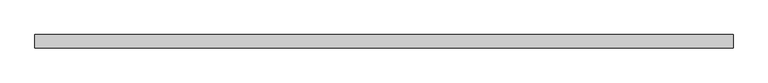
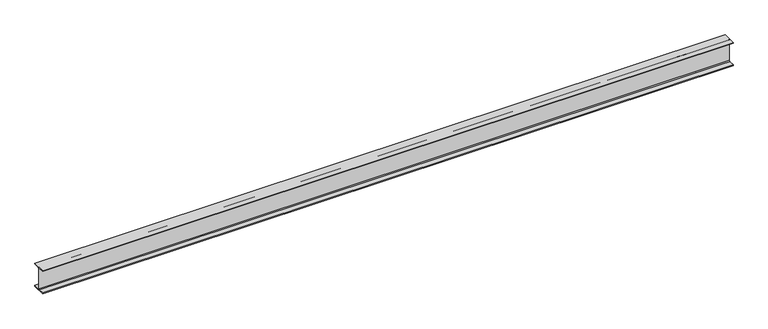
"""IFC4 building model written with IfcOpenShell, lengths in millimetres: beam geometry, Old_Steel Beam_H-KSD3502 : H_SB_ASB_H-300×300x10x15."""

from ifc_helpers import new_model, si_unit, point, frame, frame_2d, origin, place, context, project, spatial, polyline, circle_curve, trimmed, segment, composite_curve, outline, extrude, source, transform, mapped, element, save


def beam_082897f1(model_context):
    return source(origin(), model_context, "Body", "SweptSolid", [
        extrude(outline(composite_curve([segment(polyline([(82.5, -141.5), (82.5, -151.7), (-82.5, -151.7), (-82.5, -141.5), (-11.9, -141.5)]), True, "CONTINUOUS"), segment(trimmed(circle_curve(frame_2d((-11.9, -132.6)), 8.9), [point((-11.9, -141.5))], [point((-3.0, -132.6))], True, "CARTESIAN"), True, "CONTINUOUS"), segment(polyline([(-3.0, -132.6), (-3.0, 132.6)]), True, "CONTINUOUS"), segment(trimmed(circle_curve(frame_2d((-11.9, 132.6)), 8.9), [point((-3.0, 132.6))], [point((-11.9, 141.5))], True, "CARTESIAN"), True, "CONTINUOUS"), segment(polyline([(-11.9, 141.5), (-82.5, 141.5), (-82.5, 151.7), (82.5, 151.7), (82.5, 141.5), (11.9, 141.5)]), True, "CONTINUOUS"), segment(trimmed(circle_curve(frame_2d((11.9, 132.6)), 8.9), [point((11.9, 141.5))], [point((3.0, 132.6))], True, "CARTESIAN"), True, "CONTINUOUS"), segment(polyline([(3.0, 132.6), (3.0, -132.6)]), True, "CONTINUOUS"), segment(trimmed(circle_curve(frame_2d((11.9, -132.6)), 8.9), [point((3.0, -132.6))], [point((11.9, -141.5))], True, "CARTESIAN"), True, "CONTINUOUS"), segment(polyline([(11.9, -141.5), (82.5, -141.5)]), True, "CONTINUOUS")], self_intersect=False)), frame((-4272.9251782, 0.0, 0.0), z_axis=(1.0, 0.0, 0.0), x_axis=(0.0, 1.0, 0.0)), (0.0, 0.0, 1.0), 8596.9210734),
    ])


if __name__ == "__main__":
    model = new_model("IFC4")
    model_context = context("Model", 3, world=origin())
    ifc_project = project(units=[si_unit("LENGTHUNIT", "METRE", prefix="MILLI")], contexts=[model_context])
    site = spatial("IfcSite", under=ifc_project)
    building = spatial("IfcBuilding", under=site)
    placement = place(None, origin())
    beam_shape = beam_082897f1(model_context)
    element("IfcBeam", 1, ObjectType="Old_Steel Beam_H-KSD3502 : H_SB_ASB_H-300×300x10x15", at=placement, inside=building, context=model_context, shape_type="MappedRepresentation", body=[
        mapped(beam_shape, transform((0.0, 0.0, 0.0), x_axis=(1.0, 0.0, 0.0), y_axis=(0.0, 1.0, 0.0), z_axis=(0.0, 0.0, 1.0))),
    ])
    save(model, "model.ifc")

# Revit data of these elements
# Type "Old_Steel Beam_H-KSD3502 : H_SB_ASB_H-300×300x10x15"
#   Width = 30.0 cm
#   Web Thickness = 1.0 cm
#   Web Fillet = 1.8 cm
#   Warping Constant = 1370670.0 cm⁶
#   Torsional Moment of Inertia = 77.00 cm⁴
#   Torsional Modulus = 1.0 cm³
#   Section Area = 119.8 cm²
#   Plastic Modulus weak axis = 684.0 cm³
#   Plastic Modulus strong axis = 1500.0 cm³
#   Perimeter = 1.75 m²/m
#   Nominal Weight = 94.00 kgf/m
#   Moment of Inertia weak axis = 6750.00 cm⁴
#   Moment of Inertia strong axis = 20400.00 cm⁴
#   Height = 30.0 cm
#   Flange Thickness = 1.5 cm
#   Elastic Modulus weak axis = 450.0 cm³
#   Elastic Modulus strong axis = 1360.0 cm³
#   Centroid Vertical = 15.0 cm
#   Centroid Horizontal = 15.0 cm
#   Length [instance default] = 1.5240 m
#   Structural Material [instance default] = Steel, 45-345
#   Assembly Code = ""
# Element 1 (IfcBeam, "Old_Steel Beam_H-KSD3502 : H_SB_ASB_H-300×300x10x15")
#   Structural Material = none
# Materials
#   "Steel, 45-345": class "Metal", colour RGB 189 187 185, transparency 0, Description = "Steel 345 MPa", Cost = 0
